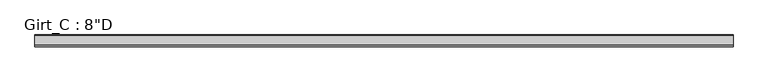
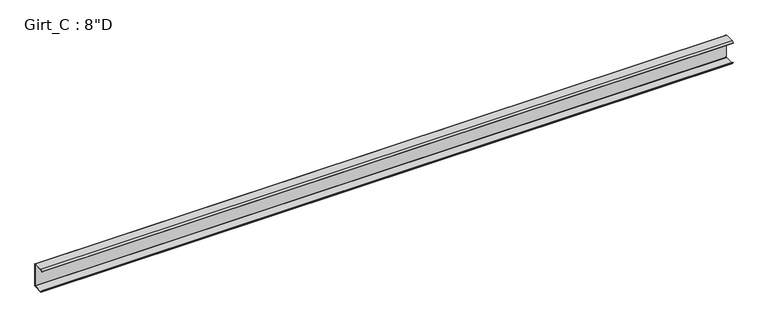
"""IFC4 building model written with IfcOpenShell, lengths in millimetres: beam geometry."""

import ifcopenshell
import ifcopenshell.guid

model = None  # the IFC model being written
_history = None  # IfcOwnerHistory: only IFC2X3 demands one
_inside = {}  # id of a spatial element -> (the spatial element, [elements in it])
_under = {}  # id of a project, library or spatial element -> (it, [spatial elements below it])
_declared = {}  # id of a project -> (the project, [libraries it declares])
_typed = {}  # id of a type object -> (the type object, [elements of that type])
_made_of = {}  # id of a material, layer set ... -> (it, [elements and type objects made of it])


def new_model(schema):
    """Start an empty IFC model of exactly this schema.

    Asked for "IFC4X3", IfcOpenShell would pick the latest addendum, in which some entities
    have other attributes; the version numbers below select the first issue.
    IFC2X3 requires an IfcOwnerHistory on every rooted entity: one is made here for all.
    """
    global model, _history
    if schema == "IFC4X3":
        model = ifcopenshell.file(schema_version=(4, 3, 0, 0))
    else:
        model = ifcopenshell.file(schema=schema)
    _inside.clear()
    _under.clear()
    _declared.clear()
    _typed.clear()
    _made_of.clear()
    _history = None
    if model.schema == "IFC2X3":
        org = make("IfcOrganization", Name="unknown")
        user = make(
            "IfcPersonAndOrganization",
            ThePerson=make("IfcPerson", FamilyName="unknown"),
            TheOrganization=org,
        )
        app = make(
            "IfcApplication",
            ApplicationDeveloper=org,
            Version="unknown",
            ApplicationFullName="unknown",
            ApplicationIdentifier="unknown",
        )
        _history = make(
            "IfcOwnerHistory",
            OwningUser=user,
            OwningApplication=app,
            ChangeAction="ADDED",
            CreationDate=0,
        )
    return model


def make(cls, **values):
    """One entity of the class cls with the attributes given. An attribute that is None is left unset."""
    return model.create_entity(
        cls, **{name: value for name, value in values.items() if value is not None}
    )


def rooted(cls, **values):
    """An entity with a GlobalId (a new one), such as an element, a storey or a relation."""
    return make(cls, GlobalId=ifcopenshell.guid.new(), OwnerHistory=_history, **values)


def si_unit(unit_type, name, prefix=None):
    """IfcSIUnit, for example si_unit("LENGTHUNIT", "METRE", prefix="MILLI")."""
    return make("IfcSIUnit", UnitType=unit_type, Prefix=prefix, Name=name)


def assignment(units):
    """IfcUnitAssignment: the units of a project."""
    return None if units is None else make("IfcUnitAssignment", Units=units)


def point(xyz):
    """IfcCartesianPoint."""
    return None if xyz is None else make("IfcCartesianPoint", Coordinates=xyz)


def direction(xyz):
    """IfcDirection."""
    return None if xyz is None else make("IfcDirection", DirectionRatios=xyz)


def frame(location, z_axis=None, x_axis=None):
    """IfcAxis2Placement3D, a coordinate frame: its origin and axes. An axis left out is left unset."""
    return make(
        "IfcAxis2Placement3D",
        Location=point(location),
        Axis=direction(z_axis),
        RefDirection=direction(x_axis),
    )


def frame_2d(location, x_axis=None):
    """IfcAxis2Placement2D, a coordinate frame in the plane: its origin and x axis."""
    return make(
        "IfcAxis2Placement2D", Location=point(location), RefDirection=direction(x_axis)
    )


def origin():
    """The frame at (0, 0, 0) with its axes left unset."""
    return frame((0.0, 0.0, 0.0))


def place(relative_to, where):
    """IfcLocalPlacement: puts the frame where relative to a parent placement (None: the world)."""
    return make(
        "IfcLocalPlacement", PlacementRelTo=relative_to, RelativePlacement=where
    )


def context(
    kind, dimensions, precision=None, world=None, true_north=None, identifier=None
):
    """IfcGeometricRepresentationContext, for example the 3D "Model" context."""
    return make(
        "IfcGeometricRepresentationContext",
        ContextIdentifier=identifier,
        ContextType=kind,
        CoordinateSpaceDimension=dimensions,
        Precision=precision,
        WorldCoordinateSystem=world,
        TrueNorth=true_north,
    )


def project(units=None, contexts=None):
    """IfcProject with its units and contexts."""
    return rooted(
        "IfcProject",
        Name="project",
        RepresentationContexts=contexts,
        UnitsInContext=assignment(units),
    )


def spatial(cls, under=None, at=None, **own):
    """A site, building, storey or space (cls), placed at a placement, below another one or the project."""
    s = rooted(cls, ObjectPlacement=at, **own)
    if under is not None:
        _under.setdefault(under.id(), (under, []))[1].append(s)
    return s


def polyline(points):
    """IfcPolyline through the points."""
    return make("IfcPolyline", Points=[point(p) for p in points])


def circle_curve(where, radius):
    """IfcCircle in the frame where."""
    return make("IfcCircle", Position=where, Radius=radius)


def trimmed(basis, trim1, trim2, sense, master):
    """IfcTrimmedCurve: the piece of a basis curve between two trims."""
    return make(
        "IfcTrimmedCurve",
        BasisCurve=basis,
        Trim1=trim1,
        Trim2=trim2,
        SenseAgreement=sense,
        MasterRepresentation=master,
    )


def segment(curve, same_sense, transition):
    """IfcCompositeCurveSegment."""
    return make(
        "IfcCompositeCurveSegment",
        Transition=transition,
        SameSense=same_sense,
        ParentCurve=curve,
    )


def composite_curve(segments, self_intersect=None):
    """IfcCompositeCurve: segments joined end to end."""
    return make("IfcCompositeCurve", Segments=segments, SelfIntersect=self_intersect)


def outline(outer, holes=None, kind="AREA"):
    """IfcArbitraryClosedProfileDef: a profile drawn as a closed curve; with holes, ...WithVoids."""
    if holes is None:
        return make("IfcArbitraryClosedProfileDef", ProfileType=kind, OuterCurve=outer)
    return make(
        "IfcArbitraryProfileDefWithVoids",
        ProfileType=kind,
        OuterCurve=outer,
        InnerCurves=holes,
    )


def extrude(swept, where, along, depth):
    """IfcExtrudedAreaSolid: the profile swept, set in the frame where, extruded along a direction by depth."""
    return make(
        "IfcExtrudedAreaSolid",
        SweptArea=swept,
        Position=where,
        ExtrudedDirection=direction(along),
        Depth=depth,
    )


def shape(context_of_items, identifier, shape_type, items):
    """IfcShapeRepresentation: the items that make up one representation, for example the "Body"."""
    return make(
        "IfcShapeRepresentation",
        ContextOfItems=context_of_items,
        RepresentationIdentifier=identifier,
        RepresentationType=shape_type,
        Items=items,
    )


def source(mapping_origin, context_of_items, identifier, shape_type, items):
    """IfcRepresentationMap: a shape defined once, which mapped items show again and again."""
    return make(
        "IfcRepresentationMap",
        MappingOrigin=mapping_origin,
        MappedRepresentation=shape(context_of_items, identifier, shape_type, items),
    )


def transform(
    local_origin,
    x_axis=None,
    y_axis=None,
    z_axis=None,
    scale=None,
    scale2=None,
    scale3=None,
    uniform=True,
):
    """IfcCartesianTransformationOperator3D, or its non-uniform kind. x_axis, y_axis, z_axis: its Axis1, 2, 3."""
    if uniform:
        return make(
            "IfcCartesianTransformationOperator3D",
            Axis1=direction(x_axis),
            Axis2=direction(y_axis),
            LocalOrigin=point(local_origin),
            Scale=scale,
            Axis3=direction(z_axis),
        )
    return make(
        "IfcCartesianTransformationOperator3DnonUniform",
        Axis1=direction(x_axis),
        Axis2=direction(y_axis),
        LocalOrigin=point(local_origin),
        Scale=scale,
        Axis3=direction(z_axis),
        Scale2=scale2,
        Scale3=scale3,
    )


def mapped(mapping_source, mapping_target):
    """IfcMappedItem: shows the shape of a source again, moved by a transform."""
    return make(
        "IfcMappedItem", MappingSource=mapping_source, MappingTarget=mapping_target
    )


def made_of(thing, what):
    """Note that an element or type object is made of a material, layer set ...; save() writes the relation."""
    if what is not None:
        _made_of.setdefault(what.id(), (what, []))[1].append(thing)
    return thing


def element(
    cls,
    number,
    at=None,
    inside=None,
    cuts=None,
    type_object=None,
    material=None,
    context=None,
    identifier="Body",
    shape_type=None,
    held_by="IfcProductDefinitionShape",
    body=None,
    shapes=None,
    **own,
):
    """One element of the class cls, such as IfcWall. Its Tag is "e" and its number.

    at: its placement. inside: the storey or other place that contains it. cuts: it is an
    opening in that element (IfcRelVoidsElement). A single representation is given by context,
    identifier, shape_type and body (its items); several are given by shapes. held_by: the class
    of the entity that holds the representations. save() writes the other relations.
    """
    e = rooted(cls, Tag="e%d" % number, ObjectPlacement=at, **own)
    if body is not None:
        shapes = [shape(context, identifier, shape_type, body)]
    if shapes is not None:
        e.Representation = make(held_by, Representations=shapes)
    if inside is not None:
        _inside.setdefault(inside.id(), (inside, []))[1].append(e)
    if cuts is not None:
        rooted(
            "IfcRelVoidsElement", RelatingBuildingElement=cuts, RelatedOpeningElement=e
        )
    if type_object is not None:
        _typed.setdefault(type_object.id(), (type_object, []))[1].append(e)
    return made_of(e, material)


def aggregate(whole, parts):
    """IfcRelAggregates: a whole, such as a stair, and the parts it consists of."""
    return rooted("IfcRelAggregates", RelatingObject=whole, RelatedObjects=parts)


def save(model, path):
    """Write the relations noted so far, then the file.

    IfcRelAggregates (storeys below a building ...), IfcRelContainedInSpatialStructure (elements
    in a storey), IfcRelDefinesByType, IfcRelAssociatesMaterial and IfcRelDeclares: one each for
    every whole, place, type object, material and project.
    """
    for whole, parts in _under.values():
        aggregate(whole, parts)
    for where, things in _inside.values():
        rooted(
            "IfcRelContainedInSpatialStructure",
            RelatedElements=things,
            RelatingStructure=where,
        )
    for kind, things in _typed.values():
        rooted("IfcRelDefinesByType", RelatedObjects=things, RelatingType=kind)
    for what, things in _made_of.values():
        rooted("IfcRelAssociatesMaterial", RelatedObjects=things, RelatingMaterial=what)
    for by, libraries in _declared.values():
        rooted("IfcRelDeclares", RelatingContext=by, RelatedDefinitions=libraries)
    model.write(path)


def beam_6fd188a8(model_context):
    return source(origin(), model_context, "Body", "SweptSolid", [
        extrude(outline(composite_curve([segment(polyline([(-87.5109375, 101.6), (-3.3734375, 101.6)]), True, "CONTINUOUS"), segment(trimmed(circle_curve(frame_2d((-3.3734375, 96.8375)), 4.7625), [point((-3.3734375, 101.6))], [point((1.3890625, 96.8375))], False, "CARTESIAN"), True, "CONTINUOUS"), segment(polyline([(1.3890625, 96.8375), (1.3890625, -96.8375)]), True, "CONTINUOUS"), segment(trimmed(circle_curve(frame_2d((-3.3734375, -96.8375)), 4.7625), [point((1.3890625, -96.8375))], [point((-3.3734375, -101.6))], False, "CARTESIAN"), True, "CONTINUOUS"), segment(polyline([(-3.3734375, -101.6), (-87.5109375, -101.6), (-99.7792647, -86.979177), (-97.6510975, -85.1934327), (-86.2154765, -98.821875), (-3.2694106, -98.821875)]), True, "CONTINUOUS"), segment(trimmed(circle_curve(frame_2d((-3.3748024, -96.8389339)), 1.9857399), [point((-3.2694106, -98.821875))], [point((-1.3890625, -96.8389339))], True, "CARTESIAN"), True, "CONTINUOUS"), segment(polyline([(-1.3890625, -96.8389339), (-1.3890625, 96.8381931)]), True, "CONTINUOUS"), segment(trimmed(circle_curve(frame_2d((-3.3741066, 96.8381931)), 1.9850441), [point((-1.3890625, 96.8381931))], [point((-3.3005807, 98.821875))], True, "CARTESIAN"), True, "CONTINUOUS"), segment(polyline([(-3.3005807, 98.821875), (-86.2154765, 98.821875), (-97.6278742, 85.221109), (-99.7560415, 87.0068534), (-87.5109375, 101.6)]), True, "CONTINUOUS")], self_intersect=False)), frame((-3051.175, 0.0, 0.0), z_axis=(1.0, 0.0, 0.0), x_axis=(0.0, 1.0, 0.0)), (0.0, 0.0, 1.0), 5864.225),
    ])


if __name__ == "__main__":
    model = new_model("IFC4")
    model_context = context("Model", 3, world=origin())
    ifc_project = project(units=[si_unit("LENGTHUNIT", "METRE", prefix="MILLI")], contexts=[model_context])
    site = spatial("IfcSite", under=ifc_project)
    building = spatial("IfcBuilding", under=site)
    placement = place(None, origin())
    beam_shape = beam_6fd188a8(model_context)
    element("IfcBeam", 1, ObjectType="Girt_C : 8\"D", at=placement, inside=building, context=model_context, shape_type="MappedRepresentation", body=[
        mapped(beam_shape, transform((0.0, 0.0, 0.0), x_axis=(1.0, 0.0, 0.0), y_axis=(0.0, 1.0, 0.0), z_axis=(0.0, 0.0, 1.0))),
    ])
    save(model, "model.ifc")

# Revit data of these elements
# Type "Girt_C : 8\"D"
#   half leg = 0' - 1 3/4"
#   Web_Thickness = 0' - 0 7/64"
#   Length [instance default] = 10' - 0"
#   Leg_1 = 0' - 3 1/2"
#   Height = 0' - 8"
#   Structural Material [instance default] = none
# Element 1 (IfcBeam, "Girt_C : 8\"D")
#   Structural Material = CEE' SECTION (8.0x3.5C - SEE STRUCT. DWGS)
#   Materials on its faces: "CEE' SECTION (8.0x3.5C - SEE STRUCT. DWGS)"
# Materials
#   "CEE' SECTION (8.0x3.5C - SEE STRUCT. DWGS)": class "Metal", colour RGB 137 146 153, transparency 0, Description = "Steel, mill finish", Cost = 0
